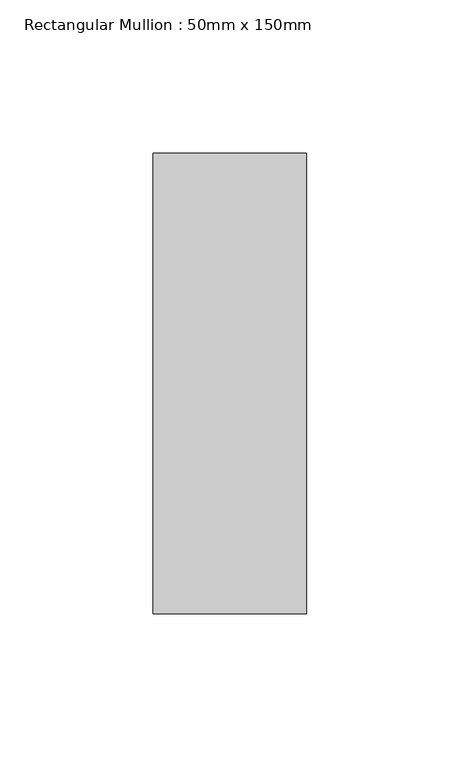
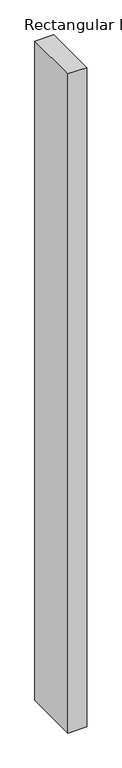
"""IFC4 building model written with IfcOpenShell, lengths in millimetres: member geometry, Rectangular Mullion : 50mm x 150mm."""

from ifc_helpers import new_model, si_unit, frame, origin, place, context, project, spatial, polyline, outline, extrude, source, transform, mapped, element, save


def rectangular_mullion_50mm_x_150mm_aaee7d48(model_context):
    return source(origin(), model_context, "Body", "SweptSolid", [
        extrude(outline(polyline([(0.0, 75.0), (0.0, -75.0), (-50.0, -75.0), (-50.0, 75.0), (0.0, 75.0)])), frame((0.0, 0.0, -1830.0), z_axis=(0.0, 0.0, 1.0), x_axis=(1.0, 0.0, 0.0)), (0.0, 0.0, 1.0), 1830.0),
    ])


if __name__ == "__main__":
    model = new_model("IFC4")
    model_context = context("Model", 3, world=origin())
    ifc_project = project(units=[si_unit("LENGTHUNIT", "METRE", prefix="MILLI")], contexts=[model_context])
    site = spatial("IfcSite", under=ifc_project)
    building = spatial("IfcBuilding", under=site)
    placement = place(None, origin())
    rectangular_mullion_50mm_x_150mm_shape = rectangular_mullion_50mm_x_150mm_aaee7d48(model_context)
    element("IfcMember", 1, ObjectType="Rectangular Mullion : 50mm x 150mm", at=placement, inside=building, context=model_context, shape_type="MappedRepresentation", body=[
        mapped(rectangular_mullion_50mm_x_150mm_shape, transform((0.0, 0.0, 0.0), x_axis=(1.0, 0.0, 0.0), y_axis=(0.0, 1.0, 0.0), z_axis=(0.0, 0.0, 1.0))),
    ])
    save(model, "model.ifc")

# Revit data of these elements
# Type "Rectangular Mullion : 50mm x 150mm"
#   built-in parameter 1007304 = 0.492126 (stored number, unit not read)
#   built-in parameter 1007301 = 0.082021 (stored number, unit not read)
#   built-in parameter 1007300 = 0.082021 (stored number, unit not read)
# Element 1 (IfcMember, "Rectangular Mullion : 50mm x 150mm")
#   Materials on its faces: "Aluminum"
# Materials
#   "Aluminum": class "Metal", colour RGB 244 244 244, transparency 0, Description = "Aluminum 6061", Cost = 0
